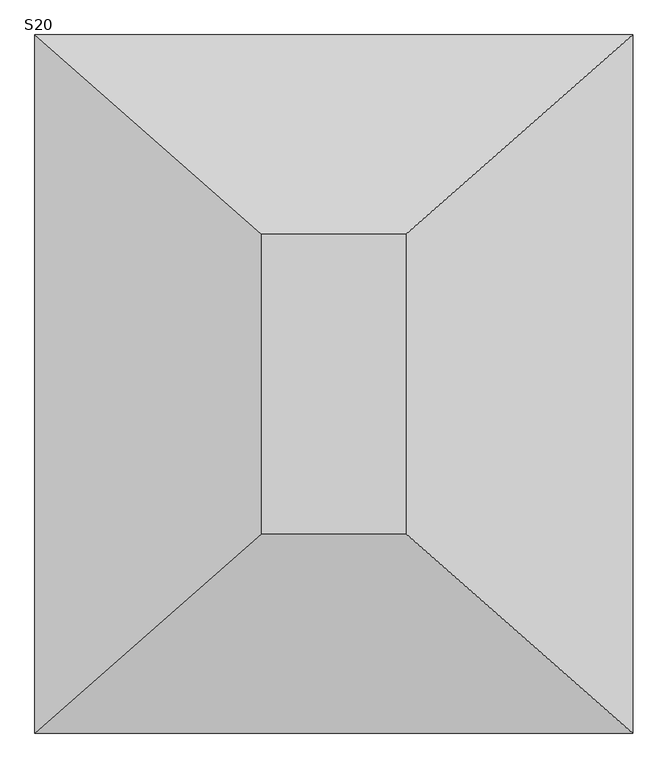
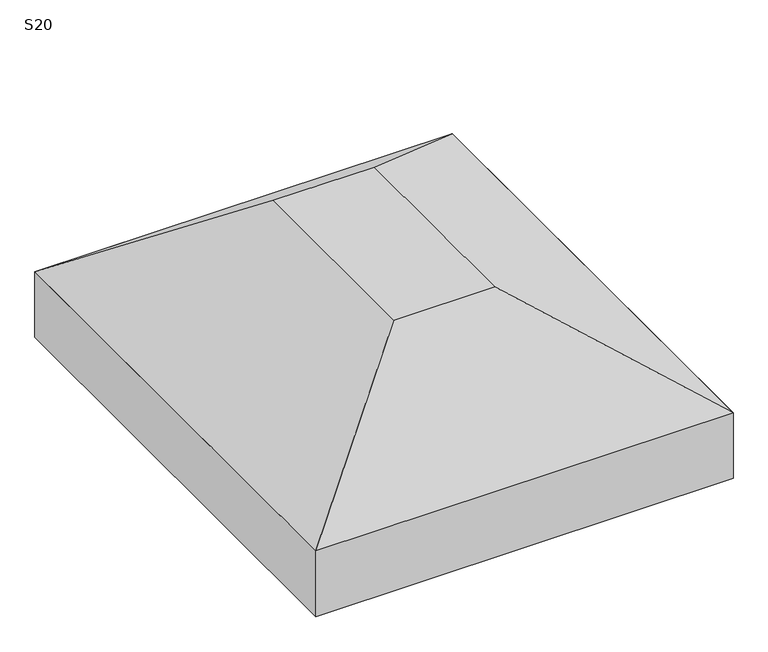
"""IFC4 building model written with IfcOpenShell, lengths in millimetres: fastener geometry, TQS - Sapata : S20."""

from ifc_helpers import new_model, si_unit, frame, origin, place, context, project, spatial, polyline, outline, extrude, faceted_brep, source, transform, mapped, element, save


def s20_c409a0c5(model_context):
    return source(origin(), model_context, "Body", "SolidModel", [
        faceted_brep([(-55.0, 100.0, 0.0), (-345.0, 100.0, 0.0), (-345.0, -500.0, 0.0), (-55.0, -500.0, 0.0), (400.0, 500.0, -300.0), (400.0, -900.0, -300.0), (-800.0, -900.0, -300.0), (-800.0, 500.0, -300.0)], [[[0, 1, 2, 3]], [[4, 5, 6, 7]], [[4, 7, 1, 0]], [[7, 6, 2, 1]], [[6, 5, 3, 2]], [[5, 4, 0, 3]]]),
        extrude(outline(polyline([(400.0, 500.0), (400.0, -900.0), (-800.0, -900.0), (-800.0, 500.0), (400.0, 500.0)])), frame((0.0, 0.0, -500.0), z_axis=(0.0, 0.0, 1.0), x_axis=(1.0, 0.0, 0.0)), (0.0, 0.0, 1.0), 200.0),
    ])


if __name__ == "__main__":
    model = new_model("IFC4")
    model_context = context("Model", 3, world=origin())
    ifc_project = project(units=[si_unit("LENGTHUNIT", "METRE", prefix="MILLI")], contexts=[model_context])
    site = spatial("IfcSite", under=ifc_project)
    building = spatial("IfcBuilding", under=site)
    placement = place(None, origin())
    s20_shape = s20_c409a0c5(model_context)
    element("IfcFastener", 1, ObjectType="TQS - Sapata : S20", at=placement, inside=building, context=model_context, shape_type="MappedRepresentation", body=[
        mapped(s20_shape, transform((0.0, 0.0, 0.0), x_axis=(1.0, 0.0, 0.0), y_axis=(0.0, 1.0, 0.0), z_axis=(0.0, 0.0, 1.0))),
    ])
    save(model, "model.ifc")

# Revit data of these elements
# Type "TQS - Sapata : S20"
#   TY = 0.60 m
#   TX = 0.29 m
#   HS = 0.50 m
#   H0 = 0.20 m
#   EXCYABS = 0.70 m
#   EXCY = 0.00 m
#   EXCXABS = 0.60 m
#   EXCX = 0.00 m
#   DIMY = 1.40 m
#   DIMX = 1.20 m
#   Material estrutural = Concreto - Concreto concretado no local
#   Width = 0
#   Length = 0
# Element 1 (IfcFastener, "TQS - Sapata : S20")
#   Materials on its faces: "Concreto - Concreto concretado no local"
# Materials
#   "Concreto - Concreto concretado no local": class "Concreto", colour RGB 192 192 192, transparency 0
